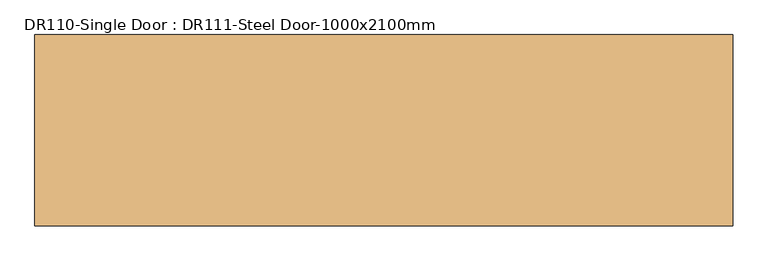
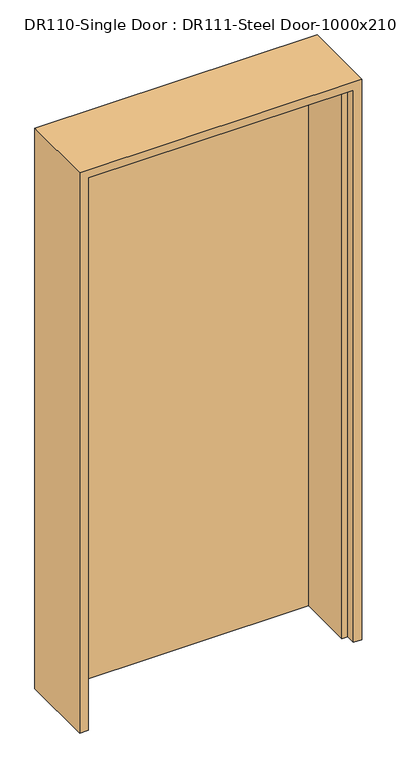
"""IFC4 building model written with IfcOpenShell, lengths in millimetres: door geometry, DR110-Single Door : DR111-Steel Door-1000x2100mm."""

import ifcopenshell
import ifcopenshell.guid

model = None  # the IFC model being written
_history = None  # IfcOwnerHistory: only IFC2X3 demands one
_inside = {}  # id of a spatial element -> (the spatial element, [elements in it])
_under = {}  # id of a project, library or spatial element -> (it, [spatial elements below it])
_declared = {}  # id of a project -> (the project, [libraries it declares])
_typed = {}  # id of a type object -> (the type object, [elements of that type])
_made_of = {}  # id of a material, layer set ... -> (it, [elements and type objects made of it])


def new_model(schema):
    """Start an empty IFC model of exactly this schema.

    Asked for "IFC4X3", IfcOpenShell would pick the latest addendum, in which some entities
    have other attributes; the version numbers below select the first issue.
    IFC2X3 requires an IfcOwnerHistory on every rooted entity: one is made here for all.
    """
    global model, _history
    if schema == "IFC4X3":
        model = ifcopenshell.file(schema_version=(4, 3, 0, 0))
    else:
        model = ifcopenshell.file(schema=schema)
    _inside.clear()
    _under.clear()
    _declared.clear()
    _typed.clear()
    _made_of.clear()
    _history = None
    if model.schema == "IFC2X3":
        org = make("IfcOrganization", Name="unknown")
        user = make(
            "IfcPersonAndOrganization",
            ThePerson=make("IfcPerson", FamilyName="unknown"),
            TheOrganization=org,
        )
        app = make(
            "IfcApplication",
            ApplicationDeveloper=org,
            Version="unknown",
            ApplicationFullName="unknown",
            ApplicationIdentifier="unknown",
        )
        _history = make(
            "IfcOwnerHistory",
            OwningUser=user,
            OwningApplication=app,
            ChangeAction="ADDED",
            CreationDate=0,
        )
    return model


def make(cls, **values):
    """One entity of the class cls with the attributes given. An attribute that is None is left unset."""
    return model.create_entity(
        cls, **{name: value for name, value in values.items() if value is not None}
    )


def rooted(cls, **values):
    """An entity with a GlobalId (a new one), such as an element, a storey or a relation."""
    return make(cls, GlobalId=ifcopenshell.guid.new(), OwnerHistory=_history, **values)


def si_unit(unit_type, name, prefix=None):
    """IfcSIUnit, for example si_unit("LENGTHUNIT", "METRE", prefix="MILLI")."""
    return make("IfcSIUnit", UnitType=unit_type, Prefix=prefix, Name=name)


def assignment(units):
    """IfcUnitAssignment: the units of a project."""
    return None if units is None else make("IfcUnitAssignment", Units=units)


def point(xyz):
    """IfcCartesianPoint."""
    return None if xyz is None else make("IfcCartesianPoint", Coordinates=xyz)


def direction(xyz):
    """IfcDirection."""
    return None if xyz is None else make("IfcDirection", DirectionRatios=xyz)


def frame(location, z_axis=None, x_axis=None):
    """IfcAxis2Placement3D, a coordinate frame: its origin and axes. An axis left out is left unset."""
    return make(
        "IfcAxis2Placement3D",
        Location=point(location),
        Axis=direction(z_axis),
        RefDirection=direction(x_axis),
    )


def origin():
    """The frame at (0, 0, 0) with its axes left unset."""
    return frame((0.0, 0.0, 0.0))


def origin_with_axes():
    """The frame at (0, 0, 0) with the z axis (0, 0, 1) and the x axis (1, 0, 0) written out."""
    return frame((0.0, 0.0, 0.0), z_axis=(0.0, 0.0, 1.0), x_axis=(1.0, 0.0, 0.0))


def place(relative_to, where):
    """IfcLocalPlacement: puts the frame where relative to a parent placement (None: the world)."""
    return make(
        "IfcLocalPlacement", PlacementRelTo=relative_to, RelativePlacement=where
    )


def context(
    kind, dimensions, precision=None, world=None, true_north=None, identifier=None
):
    """IfcGeometricRepresentationContext, for example the 3D "Model" context."""
    return make(
        "IfcGeometricRepresentationContext",
        ContextIdentifier=identifier,
        ContextType=kind,
        CoordinateSpaceDimension=dimensions,
        Precision=precision,
        WorldCoordinateSystem=world,
        TrueNorth=true_north,
    )


def project(units=None, contexts=None):
    """IfcProject with its units and contexts."""
    return rooted(
        "IfcProject",
        Name="project",
        RepresentationContexts=contexts,
        UnitsInContext=assignment(units),
    )


def spatial(cls, under=None, at=None, **own):
    """A site, building, storey or space (cls), placed at a placement, below another one or the project."""
    s = rooted(cls, ObjectPlacement=at, **own)
    if under is not None:
        _under.setdefault(under.id(), (under, []))[1].append(s)
    return s


def polyline(points):
    """IfcPolyline through the points."""
    return make("IfcPolyline", Points=[point(p) for p in points])


def outline(outer, holes=None, kind="AREA"):
    """IfcArbitraryClosedProfileDef: a profile drawn as a closed curve; with holes, ...WithVoids."""
    if holes is None:
        return make("IfcArbitraryClosedProfileDef", ProfileType=kind, OuterCurve=outer)
    return make(
        "IfcArbitraryProfileDefWithVoids",
        ProfileType=kind,
        OuterCurve=outer,
        InnerCurves=holes,
    )


def extrude(swept, where, along, depth):
    """IfcExtrudedAreaSolid: the profile swept, set in the frame where, extruded along a direction by depth."""
    return make(
        "IfcExtrudedAreaSolid",
        SweptArea=swept,
        Position=where,
        ExtrudedDirection=direction(along),
        Depth=depth,
    )


def faces_of(points, faces, orient=None, outer=None):
    """IfcFace entities. A face is a list of loops; a loop is a list of indices into points, from 0.

    orient and outer hold one flag for each loop. By default every Orientation is true, the
    first loop of a face is its IfcFaceOuterBound and the others are IfcFaceBound.
    """
    made = []
    for i, loops in enumerate(faces):
        bounds = []
        for j, loop in enumerate(loops):
            is_outer = j == 0 if outer is None else outer[i][j]
            bounds.append(
                make(
                    "IfcFaceOuterBound" if is_outer else "IfcFaceBound",
                    Bound=make("IfcPolyLoop", Polygon=[points[k] for k in loop]),
                    Orientation=True if orient is None else orient[i][j],
                )
            )
        made.append(make("IfcFace", Bounds=bounds))
    return made


def faceted_brep(points, faces, orient=None, outer=None, voids=None):
    """IfcFacetedBrep: a solid bounded by flat faces; with voids (closed shells), ...WithVoids."""
    shared = [point(p) for p in points]
    hull = make("IfcClosedShell", CfsFaces=faces_of(shared, faces, orient, outer))
    if voids is None:
        return make("IfcFacetedBrep", Outer=hull)
    return make(
        "IfcFacetedBrepWithVoids",
        Outer=hull,
        Voids=[
            make(cls, CfsFaces=faces_of(shared, fs, o, b)) for cls, fs, o, b in voids
        ],
    )


def shape(context_of_items, identifier, shape_type, items):
    """IfcShapeRepresentation: the items that make up one representation, for example the "Body"."""
    return make(
        "IfcShapeRepresentation",
        ContextOfItems=context_of_items,
        RepresentationIdentifier=identifier,
        RepresentationType=shape_type,
        Items=items,
    )


def source(mapping_origin, context_of_items, identifier, shape_type, items):
    """IfcRepresentationMap: a shape defined once, which mapped items show again and again."""
    return make(
        "IfcRepresentationMap",
        MappingOrigin=mapping_origin,
        MappedRepresentation=shape(context_of_items, identifier, shape_type, items),
    )


def transform(
    local_origin,
    x_axis=None,
    y_axis=None,
    z_axis=None,
    scale=None,
    scale2=None,
    scale3=None,
    uniform=True,
):
    """IfcCartesianTransformationOperator3D, or its non-uniform kind. x_axis, y_axis, z_axis: its Axis1, 2, 3."""
    if uniform:
        return make(
            "IfcCartesianTransformationOperator3D",
            Axis1=direction(x_axis),
            Axis2=direction(y_axis),
            LocalOrigin=point(local_origin),
            Scale=scale,
            Axis3=direction(z_axis),
        )
    return make(
        "IfcCartesianTransformationOperator3DnonUniform",
        Axis1=direction(x_axis),
        Axis2=direction(y_axis),
        LocalOrigin=point(local_origin),
        Scale=scale,
        Axis3=direction(z_axis),
        Scale2=scale2,
        Scale3=scale3,
    )


def mapped(mapping_source, mapping_target):
    """IfcMappedItem: shows the shape of a source again, moved by a transform."""
    return make(
        "IfcMappedItem", MappingSource=mapping_source, MappingTarget=mapping_target
    )


def made_of(thing, what):
    """Note that an element or type object is made of a material, layer set ...; save() writes the relation."""
    if what is not None:
        _made_of.setdefault(what.id(), (what, []))[1].append(thing)
    return thing


def element(
    cls,
    number,
    at=None,
    inside=None,
    cuts=None,
    type_object=None,
    material=None,
    context=None,
    identifier="Body",
    shape_type=None,
    held_by="IfcProductDefinitionShape",
    body=None,
    shapes=None,
    **own,
):
    """One element of the class cls, such as IfcWall. Its Tag is "e" and its number.

    at: its placement. inside: the storey or other place that contains it. cuts: it is an
    opening in that element (IfcRelVoidsElement). A single representation is given by context,
    identifier, shape_type and body (its items); several are given by shapes. held_by: the class
    of the entity that holds the representations. save() writes the other relations.
    """
    e = rooted(cls, Tag="e%d" % number, ObjectPlacement=at, **own)
    if body is not None:
        shapes = [shape(context, identifier, shape_type, body)]
    if shapes is not None:
        e.Representation = make(held_by, Representations=shapes)
    if inside is not None:
        _inside.setdefault(inside.id(), (inside, []))[1].append(e)
    if cuts is not None:
        rooted(
            "IfcRelVoidsElement", RelatingBuildingElement=cuts, RelatedOpeningElement=e
        )
    if type_object is not None:
        _typed.setdefault(type_object.id(), (type_object, []))[1].append(e)
    return made_of(e, material)


def aggregate(whole, parts):
    """IfcRelAggregates: a whole, such as a stair, and the parts it consists of."""
    return rooted("IfcRelAggregates", RelatingObject=whole, RelatedObjects=parts)


def save(model, path):
    """Write the relations noted so far, then the file.

    IfcRelAggregates (storeys below a building ...), IfcRelContainedInSpatialStructure (elements
    in a storey), IfcRelDefinesByType, IfcRelAssociatesMaterial and IfcRelDeclares: one each for
    every whole, place, type object, material and project.
    """
    for whole, parts in _under.values():
        aggregate(whole, parts)
    for where, things in _inside.values():
        rooted(
            "IfcRelContainedInSpatialStructure",
            RelatedElements=things,
            RelatingStructure=where,
        )
    for kind, things in _typed.values():
        rooted("IfcRelDefinesByType", RelatedObjects=things, RelatingType=kind)
    for what, things in _made_of.values():
        rooted("IfcRelAssociatesMaterial", RelatedObjects=things, RelatingMaterial=what)
    for by, libraries in _declared.values():
        rooted("IfcRelDeclares", RelatingContext=by, RelatedDefinitions=libraries)
    model.write(path)


def dr110_single_door_dr111_steel_door_1000x2100mm_d0b51d4b(model_context):
    return source(origin(), model_context, "Body", "SolidModel", [
        extrude(outline(polyline([(470.0, 137.0), (470.0, 102.0), (-470.0, 102.0), (-470.0, 137.0), (470.0, 137.0)])), origin_with_axes(), (0.0, 0.0, 1.0), 2070.0),
        faceted_brep([(470.0, 137.0, 0.0), (500.0, 137.0, 0.0), (500.0, -137.0, 0.0), (470.0, -137.0, 0.0), (470.0, -102.0, 0.0), (450.0, -102.0, 0.0), (450.0, 102.0, 0.0), (470.0, 102.0, 0.0), (470.0, 137.0, 2070.0), (-470.0, 137.0, 2070.0), (-470.0, 137.0, 0.0), (-500.0, 137.0, 0.0), (-500.0, 137.0, 2100.0), (500.0, 137.0, 2100.0), (500.0, -137.0, 2100.0), (-500.0, -137.0, 2100.0), (-500.0, -137.0, 0.0), (-470.0, -137.0, 0.0), (-470.0, -137.0, 2070.0), (470.0, -137.0, 2070.0), (470.0, -102.0, 2070.0), (-470.0, -102.0, 2070.0), (-470.0, -102.0, 0.0), (-450.0, -102.0, 0.0), (-450.0, -102.0, 2050.0), (450.0, -102.0, 2050.0), (450.0, 102.0, 2050.0), (-450.0, 102.0, 2050.0), (-450.0, 102.0, 0.0), (-470.0, 102.0, 0.0), (-470.0, 102.0, 2070.0), (470.0, 102.0, 2070.0)], [[[0, 1, 2, 3, 4, 5, 6, 7]], [[1, 0, 8, 9, 10, 11, 12, 13]], [[2, 1, 13, 14]], [[3, 2, 14, 15, 16, 17, 18, 19]], [[4, 3, 19, 20]], [[5, 4, 20, 21, 22, 23, 24, 25]], [[6, 5, 25, 26]], [[7, 6, 26, 27, 28, 29, 30, 31]], [[0, 7, 31, 8]], [[9, 30, 29, 10]], [[10, 29, 28, 23, 22, 17, 16, 11]], [[15, 12, 11, 16]], [[21, 18, 17, 22]], [[27, 24, 23, 28]], [[14, 13, 12, 15]], [[20, 19, 18, 21]], [[26, 25, 24, 27]], [[8, 31, 30, 9]]]),
    ])


if __name__ == "__main__":
    model = new_model("IFC4")
    model_context = context("Model", 3, world=origin())
    ifc_project = project(units=[si_unit("LENGTHUNIT", "METRE", prefix="MILLI")], contexts=[model_context])
    site = spatial("IfcSite", under=ifc_project)
    building = spatial("IfcBuilding", under=site)
    placement = place(None, origin())
    dr110_single_door_dr111_steel_door_1000x2100mm_shape = dr110_single_door_dr111_steel_door_1000x2100mm_d0b51d4b(model_context)
    element("IfcDoor", 1, ObjectType="DR110-Single Door : DR111-Steel Door-1000x2100mm", at=placement, inside=building, context=model_context, shape_type="MappedRepresentation", body=[
        mapped(dr110_single_door_dr111_steel_door_1000x2100mm_shape, transform((0.0, 0.0, 0.0), x_axis=(1.0, 0.0, 0.0), y_axis=(0.0, 1.0, 0.0), z_axis=(0.0, 0.0, 1.0))),
    ])
    save(model, "model.ifc")

# Revit data of these elements
# Type "DR110-Single Door : DR111-Steel Door-1000x2100mm"
#   Type Mark = ""
#   Analytic Construction = "<None>"
#   프레임 투영 외부. = 25 mm
#   프레임 투영 내부. = 25 mm
#   프레임 폭 = 75 mm
#   Height = 2100 mm
#   Width = 1000 mm
#   Define Thermal Properties by = 1
#   문 패널 = SD1 문 패널
#   문 프레임 = A04AQ098-00002_Steel Door_non FP_single
#   Function = (empty or 0)
#   Wall Closure = (empty or 0)
# Element 1 (IfcDoor, "DR110-Single Door : DR111-Steel Door-1000x2100mm")
#   Materials on its faces: "A04AQ098-00002_Steel Door_non FP_single", "SD1 문 패널"
# Materials
#   "SD1 문 패널": class "금속", colour RGB 247 247 247, transparency 0
#   "A04AQ098-00002_Steel Door_non FP_single": class "금속", colour RGB 247 247 247, transparency 0, Description = "Steel Door", W00) Work Master Code = "A04AQ098-00002", W01) Work Master_Lv1 = "Finishing Work", W02) Work Master_Lv2 = "Door & Window Work", W03) Work Master_Spec.1 = "Steel Door w/ Steel Frame", W04) Work Master_Spec.2 = "Fire Protective Rating: N/A, Single Door", W05) Work Master_Spec.3 = "w/ Hardware & Accessories", Cost = 0
